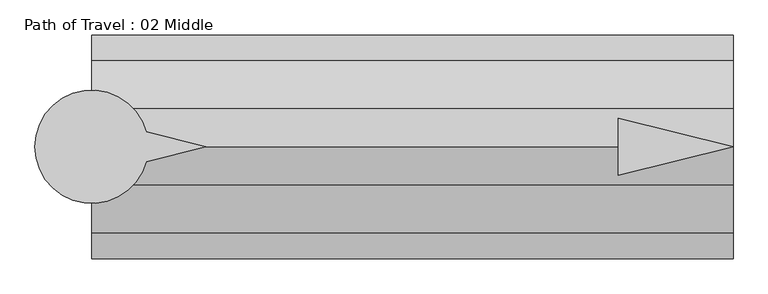
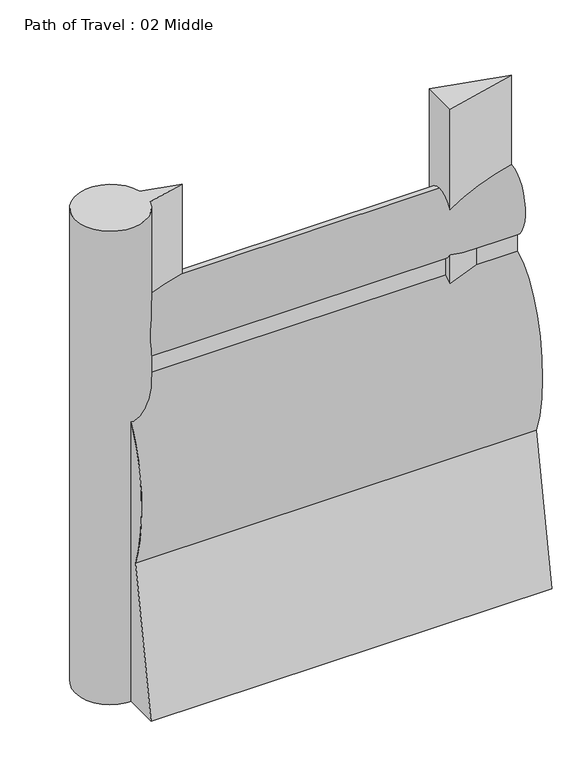
"""IFC4 building model written with IfcOpenShell, lengths in millimetres: proxy geometry, Path of Travel : 02 Middle."""

from ifc_helpers import new_model, si_unit, point, frame, frame_2d, origin, origin_with_axes, place, context, project, spatial, polyline, circle_curve, ellipse_curve, trimmed, segment, composite_curve, outline, extrude, source, transform, mapped, element, save
from ifc_brep_helpers import plane_surface, extruded_surface, advanced_brep


def path_of_travel_02_middle_e3fffb2b(model_context):
    return source(origin(), model_context, "Body", "SolidModel", [
        advanced_brep(
        [(227.5554837, 0.0, 1727.2), (227.5554837, 42.9018657, 1436.6534209), (227.5554837, 42.9018657, 1363.4763406), (227.5554837, 184.1186263, 643.4144547), (227.5554837, 297.5699544, 0.0), (227.5554837, 145.6574193, 0.0), (227.5554837, 0.0, 584.2), (227.5554837, -145.6574193, 0.0), (227.5554837, -297.5699544, 0.0), (227.5554837, -184.1186263, 643.4144547), (227.5554837, -42.9018657, 1363.4763406), (227.5554837, -42.9018657, 1436.6534209), (1934.2322282, 0.0, 1727.2), (1934.2322282, -42.9018657, 1436.6534209), (1934.2322282, -42.9018657, 1363.4763406), (1934.2322282, -184.1186263, 643.4144547), (1934.2322282, -297.5699544, 0.0), (1934.2322282, -145.6574193, 0.0), (1934.2322282, 0.0, 584.2), (1934.2322282, 145.6574193, 0.0), (1934.2322282, 297.5699544, 0.0), (1934.2322282, 184.1186263, 643.4144547), (1934.2322282, 42.9018657, 1363.4763406), (1934.2322282, 42.9018657, 1436.6534209)],
        [
            (0, 1, ellipse_curve(frame((227.5554837, 0.0, 1574.8), z_axis=(-1.0, 0.0, 0.0), x_axis=(0.0, 0.0, 1.0)), 152.4, 101.6)),
            (1, 2),
            (2, 3, ellipse_curve(frame((227.5554837, 0.0, 914.4), z_axis=(-1.0, 0.0, 0.0), x_axis=(0.0, 0.0, -1.0)), 457.2, 228.6)),
            (3, 4),
            (4, 5),
            (5, 6),
            (6, 7),
            (7, 8),
            (8, 9),
            (9, 10, ellipse_curve(frame((227.5554837, 0.0, 914.4), z_axis=(-1.0, 0.0, 0.0), x_axis=(0.0, 0.0, -1.0)), 457.2, 228.6)),
            (10, 11),
            (11, 0, ellipse_curve(frame((227.5554837, 0.0, 1574.8), z_axis=(-1.0, 0.0, 0.0), x_axis=(0.0, 0.0, 1.0)), 152.4, 101.6)),
            (12, 13, ellipse_curve(frame((1934.2322282, 0.0, 1574.8), z_axis=(1.0, 0.0, 0.0), x_axis=(0.0, 0.0, 1.0)), 152.4, 101.6)),
            (13, 14),
            (14, 15, ellipse_curve(frame((1934.2322282, 0.0, 914.4), z_axis=(1.0, 0.0, 0.0), x_axis=(0.0, 0.0, -1.0)), 457.2, 228.6)),
            (15, 16),
            (16, 17),
            (17, 18),
            (18, 19),
            (19, 20),
            (20, 21),
            (21, 22, ellipse_curve(frame((1934.2322282, 0.0, 914.4), z_axis=(1.0, 0.0, 0.0), x_axis=(0.0, 0.0, -1.0)), 457.2, 228.6)),
            (22, 23),
            (23, 12, ellipse_curve(frame((1934.2322282, 0.0, 1574.8), z_axis=(1.0, 0.0, 0.0), x_axis=(0.0, 0.0, 1.0)), 152.4, 101.6)),
            (0, 12),
            (23, 1),
            (22, 2),
            (21, 3),
            (20, 4),
            (19, 5),
            (18, 6),
            (17, 7),
            (16, 8),
            (15, 9),
            (14, 10),
            (13, 11),
        ],
        [
            plane_surface(frame((227.5554837, 0.0, 0.0), z_axis=(-1.0, 0.0, 0.0), x_axis=(0.0, 0.0, 1.0))),
            plane_surface(frame((1934.2322282, 0.0, 0.0), z_axis=(1.0, 0.0, 0.0), x_axis=(0.0, 0.0, 1.0))),
            extruded_surface(trimmed(ellipse_curve(frame((1934.2322282, 0.0, 1574.8), z_axis=(-1.0, 0.0, 0.0), x_axis=(0.0, 0.0, 1.0)), 152.4, 101.6), [point((1934.2322282, 0.0, 1727.2))], [point((1934.2322282, 42.9018657, 1436.6534209))], True, "CARTESIAN"), (-1706.6767445, 0.0, 0.0), 1706.6767445),
            plane_surface(frame((227.5554837, 42.9018657, 1436.6534209), z_axis=(0.0, 1.0, 0.0), x_axis=(1.0, 0.0, 0.0))),
            extruded_surface(trimmed(ellipse_curve(frame((1934.2322282, 0.0, 914.4), z_axis=(-1.0, 0.0, 0.0), x_axis=(0.0, 0.0, -1.0)), 457.2, 228.6), [point((1934.2322282, 42.9018657, 1363.4763406))], [point((1934.2322282, 184.1186263, 643.4144547))], True, "CARTESIAN"), (-1706.6767445, 0.0, 0.0), 1706.6767445),
            plane_surface(frame((227.5554837, 184.1186263, 643.4144547), z_axis=(0.0, 0.9848077530122078, 0.1736481776669322), x_axis=(1.0, 0.0, 0.0))),
            plane_surface(frame((227.5554837, 297.5699544, 0.0), z_axis=(0.0, 0.0, -1.0), x_axis=(1.0, 0.0, 0.0))),
            plane_surface(frame((227.5554837, 145.6574193, 0.0), z_axis=(0.0, -0.9702957262760199, -0.2419218955995739), x_axis=(1.0, 0.0, 0.0))),
            plane_surface(frame((227.5554837, 0.0, 584.2), z_axis=(0.0, 0.9702957262759961, -0.24192189559966923), x_axis=(1.0, 0.0, 0.0))),
            plane_surface(frame((227.5554837, -145.6574193, 0.0), z_axis=(0.0, 0.0, -1.0), x_axis=(1.0, 0.0, 0.0))),
            plane_surface(frame((227.5554837, -297.5699544, 0.0), z_axis=(0.0, -0.984807753012208, 0.17364817766693066), x_axis=(1.0, 0.0, 0.0))),
            extruded_surface(trimmed(ellipse_curve(frame((1934.2322282, 0.0, 914.4), z_axis=(-1.0, 0.0, 0.0), x_axis=(0.0, 0.0, -1.0)), 457.2, 228.6), [point((1934.2322282, -184.1186263, 643.4144547))], [point((1934.2322282, -42.9018657, 1363.4763406))], True, "CARTESIAN"), (-1706.6767445, 0.0, 0.0), 1706.6767445),
            plane_surface(frame((227.5554837, -42.9018657, 1363.4763406), z_axis=(0.0, -1.0, 0.0), x_axis=(1.0, 0.0, 0.0))),
            extruded_surface(trimmed(ellipse_curve(frame((1934.2322282, 0.0, 1574.8), z_axis=(-1.0, 0.0, 0.0), x_axis=(0.0, 0.0, 1.0)), 152.4, 101.6), [point((1934.2322282, -42.9018657, 1436.6534209))], [point((1934.2322282, 0.0, 1727.2))], True, "CARTESIAN"), (-1706.6767445, 0.0, 0.0), 1706.6767445),
        ],
        [
            (0, [[1, 2, 3, 4, 5, 6, 7, 8, 9, 10, 11, 12]]),
            (1, [[13, 14, 15, 16, 17, 18, 19, 20, 21, 22, 23, 24]]),
            (2, [[-1, 25, -24, 26]]),
            (3, [[-2, -26, -23, 27]]),
            (4, [[-3, -27, -22, 28]]),
            (5, [[-4, -28, -21, 29]]),
            (6, [[-5, -29, -20, 30]]),
            (7, [[-6, -30, -19, 31]]),
            (8, [[-7, -31, -18, 32]]),
            (9, [[-8, -32, -17, 33]]),
            (10, [[-9, -33, -16, 34]]),
            (11, [[-10, -34, -15, 35]]),
            (12, [[-11, -35, -14, 36]]),
            (13, [[-12, -36, -13, -25]]),
        ],
    ),
        extrude(outline(polyline([(1628.2270816, 76.2006338), (1934.2322282, 0.0), (1628.2270816, -76.2006338), (1628.2270816, 76.2006338)])), origin_with_axes(), (0.0, 0.0, 1.0), 2129.5973753),
        extrude(outline(composite_curve([segment(polyline([(372.7837828, 39.4440225), (531.182385, 0.0), (372.7837828, -39.4440225)]), True, "CONTINUOUS"), segment(trimmed(circle_curve(frame_2d((227.2200886, 0.0)), 150.8131956), [point((372.7837828, -39.4440225))], [point((372.7837828, 39.4440225))], False, "CARTESIAN"), True, "CONTINUOUS")], self_intersect=False)), origin_with_axes(), (0.0, 0.0, 1.0), 2129.5973753),
    ])


if __name__ == "__main__":
    model = new_model("IFC4")
    model_context = context("Model", 3, world=origin())
    ifc_project = project(units=[si_unit("LENGTHUNIT", "METRE", prefix="MILLI")], contexts=[model_context])
    site = spatial("IfcSite", under=ifc_project)
    building = spatial("IfcBuilding", under=site)
    placement = place(None, origin())
    path_of_travel_02_middle_shape = path_of_travel_02_middle_e3fffb2b(model_context)
    element("IfcBuildingElementProxy", 1, Name="Path of Travel : 02 Middle", ObjectType="Path of Travel : 02 Middle", at=placement, inside=building, context=model_context, shape_type="MappedRepresentation", body=[
        mapped(path_of_travel_02_middle_shape, transform((0.0, 0.0, 0.0), x_axis=(1.0, 0.0, 0.0), y_axis=(0.0, 1.0, 0.0), z_axis=(0.0, 0.0, 1.0))),
    ])
    save(model, "model.ifc")

# Revit data of these elements
# Type "Path of Travel : 02 Middle"
#   Path of Egress [instance default] = 4' - 0"
#   built-in parameter 1001306 [instance default] = 4 (stored number, unit not read)
#   Dot at Start = no
#   Arrow in Middle = yes
#   Arrow at End = no
#   Egress Path = none
# Element 1 (IfcBuildingElementProxy, "Path of Travel : 02 Middle")
#   Path of Egress = 5' - 7.192"
#   built-in parameter 1001306 = 5.59933 (stored number, unit not read)
